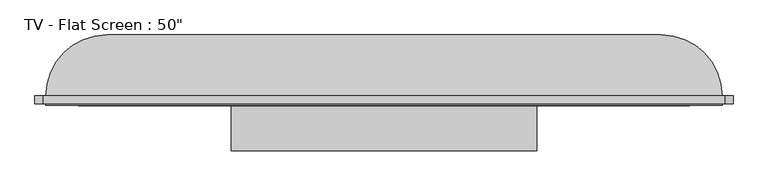
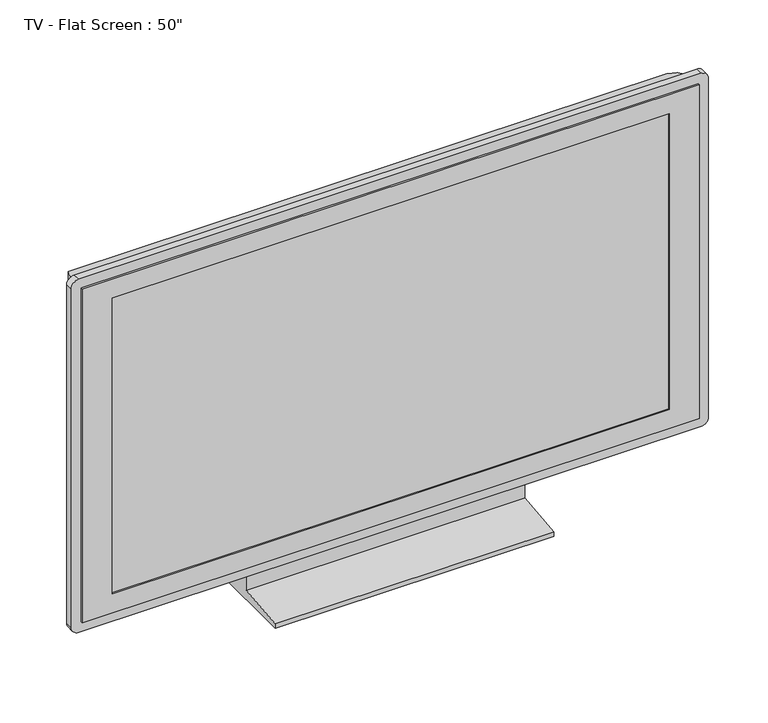
"""IFC4 building model written with IfcOpenShell, lengths in millimetres: furniture geometry."""

from ifc_helpers import new_model, si_unit, point, frame, frame_2d, origin, place, context, project, spatial, polyline, circle_curve, ellipse_curve, trimmed, segment, composite_curve, outline, extrude, faceted_brep, source, transform, mapped, element, save
from ifc_brep_helpers import plane_surface, cylinder_surface, advanced_brep


def furniture_fdf74506(model_context):
    return source(origin(), model_context, "Body", "SolidModel", [
        extrude(outline(polyline([(-51.4613764, 80.0), (-1.4613764, 80.0), (48.5386236, 0.0), (-151.4613764, 0.0), (-151.4613764, 10.0), (-51.4613764, 20.0), (-51.4613764, 80.0)])), frame((-280.6636439, 0.0, 0.0), z_axis=(1.0, 0.0, 0.0), x_axis=(0.0, 1.0, 0.0)), (0.0, 0.0, 1.0), 553.4382596),
        faceted_brep([(609.4937454, -69.4613764, 782.6751733), (-617.3827737, -69.4613764, 782.6751733), (-617.3827737, -69.4613764, 80.0), (609.4937454, -69.4613764, 80.0), (-557.3827737, -69.4613764, 742.6751733), (549.4937454, -69.4613764, 742.6751733), (549.4937454, -69.4613764, 120.0), (-557.3827737, -69.4613764, 120.0), (609.4937454, -51.4613764, 782.6751733), (609.4937454, -51.4613764, 80.0), (-617.3827737, -51.4613764, 80.0), (-617.3827737, -51.4613764, 782.6751733), (-557.3827737, -66.4613764, 742.6751733), (-557.3827737, -66.4613764, 120.0), (549.4937454, -66.4613764, 120.0), (549.4937454, -66.4613764, 742.6751733)], [[[0, 1, 2, 3], [4, 5, 6, 7]], [[8, 9, 10, 11]], [[1, 0, 8, 11]], [[2, 1, 11, 10]], [[3, 2, 10, 9]], [[0, 3, 9, 8]], [[12, 13, 14, 15]], [[12, 15, 5, 4]], [[15, 14, 6, 5]], [[14, 13, 7, 6]], [[13, 12, 4, 7]]]),
        extrude(outline(composite_curve([segment(polyline([(802.6751733, 614.4937454), (802.6751733, -622.3827737)]), True, "CONTINUOUS"), segment(trimmed(circle_curve(frame_2d((787.6751733, -622.3827737)), 15.0), [point((802.6751733, -622.3827737))], [point((787.6751733, -637.3827737))], False, "CARTESIAN"), True, "CONTINUOUS"), segment(polyline([(787.6751733, -637.3827737), (75.0, -637.3827737)]), True, "CONTINUOUS"), segment(trimmed(circle_curve(frame_2d((75.0, -622.3827737)), 15.0), [point((75.0, -637.3827737))], [point((60.0, -622.3827737))], False, "CARTESIAN"), True, "CONTINUOUS"), segment(polyline([(60.0, -622.3827737), (60.0, 614.4937454)]), True, "CONTINUOUS"), segment(trimmed(circle_curve(frame_2d((75.0, 614.4937454)), 15.0), [point((60.0, 614.4937454))], [point((75.0, 629.4937454))], False, "CARTESIAN"), True, "CONTINUOUS"), segment(polyline([(75.0, 629.4937454), (787.6751733, 629.4937454)]), True, "CONTINUOUS"), segment(trimmed(circle_curve(frame_2d((787.6751733, 614.4937454)), 15.0), [point((787.6751733, 629.4937454))], [point((802.6751733, 614.4937454))], False, "CARTESIAN"), True, "CONTINUOUS")], self_intersect=False), holes=[polyline([(782.6751733, 609.4937454), (80.0, 609.4937454), (80.0, -617.3827737), (782.6751733, -617.3827737), (782.6751733, 609.4937454)])]), frame((0.0, -66.4613764, 0.0), z_axis=(0.0, 1.0, 0.0), x_axis=(0.0, 0.0, 1.0)), (0.0, 0.0, 1.0), 15.0),
        advanced_brep(
        [(-617.3827737, -51.4613764, 80.0), (609.4937454, -51.4613764, 80.0), (609.4937454, -51.4613764, 782.6751733), (-617.3827737, -51.4613764, 782.6751733), (499.4937454, 58.5386236, 80.0), (-507.3827737, 58.5386236, 80.0), (-507.3827737, 58.5386236, 672.6751733), (499.4937454, 58.5386236, 672.6751733)],
        [
            (0, 1),
            (1, 2),
            (2, 3),
            (3, 0),
            (4, 5),
            (5, 6),
            (6, 7),
            (7, 4),
            (0, 5, circle_curve(frame((-507.3827737, -51.4613764, 80.0), z_axis=(0.0, 0.0, -1.0), x_axis=(-1.0, 0.0, 0.0)), 110.0)),
            (4, 1, circle_curve(frame((499.4937454, -51.4613764, 80.0), z_axis=(0.0, 0.0, -1.0), x_axis=(1.0, 0.0, 0.0)), 110.0)),
            (7, 2, ellipse_curve(frame((499.4937454, -51.4613764, 672.6751733), z_axis=(0.7071067811865475, 0.0, -0.7071067811865475), x_axis=(0.7071067811865474, 0.0, 0.7071067811865476)), 155.5634919, 110.0)),
            (6, 3, ellipse_curve(frame((-507.3827737, -51.4613764, 672.6751733), z_axis=(0.7071067811865475, 0.0, 0.7071067811865475), x_axis=(-0.7071067811865476, 0.0, 0.7071067811865474)), 155.5634919, 110.0)),
        ],
        [
            plane_surface(frame((-617.3827737, -51.4613764, 782.6751733), z_axis=(0.0, -1.0, 0.0), x_axis=(-1.0, 0.0, 0.0))),
            plane_surface(frame((-617.3827737, 58.5386236, 782.6751733), z_axis=(0.0, 1.0, 0.0), x_axis=(1.0, 0.0, 0.0))),
            plane_surface(frame((-617.3827737, -51.4613764, 80.0), z_axis=(0.0, 0.0, -1.0), x_axis=(0.0, 1.0, 0.0))),
            cylinder_surface(frame((499.4937454, -51.4613764, 80.0), z_axis=(0.0, 0.0, 1.0), x_axis=(1.0, 0.0, 0.0)), 110.0),
            cylinder_surface(frame((609.4937454, -51.4613764, 672.6751733), z_axis=(-1.0, 0.0, 0.0), x_axis=(0.0, 0.0, 1.0)), 110.0),
            cylinder_surface(frame((-507.3827737, -51.4613764, 782.6751733), z_axis=(0.0, 0.0, -1.0), x_axis=(-1.0, 0.0, 0.0)), 110.0),
        ],
        [
            (0, [[1, 2, 3, 4]]),
            (1, [[5, 6, 7, 8]]),
            (2, [[-1, 9, -5, 10]]),
            (3, [[11, -2, -10, -8]]),
            (4, [[-11, -7, 12, -3]]),
            (5, [[-12, -6, -9, -4]]),
        ],
    ),
    ])


if __name__ == "__main__":
    model = new_model("IFC4")
    model_context = context("Model", 3, world=origin())
    ifc_project = project(units=[si_unit("LENGTHUNIT", "METRE", prefix="MILLI")], contexts=[model_context])
    site = spatial("IfcSite", under=ifc_project)
    building = spatial("IfcBuilding", under=site)
    placement = place(None, origin())
    furniture_shape = furniture_fdf74506(model_context)
    element("IfcFurniture", 1, ObjectType="TV - Flat Screen : 50\"", at=placement, inside=building, context=model_context, shape_type="MappedRepresentation", body=[
        mapped(furniture_shape, transform((0.0, 0.0, 0.0), x_axis=(1.0, 0.0, 0.0), y_axis=(0.0, 1.0, 0.0), z_axis=(0.0, 0.0, 1.0))),
    ])
    save(model, "model.ifc")

# Revit data of these elements
# Type "TV - Flat Screen : 50\""
#   SinAng = 0' - 0.0193"
#   L = 3' - 7.57782"
#   H = 2' - 0.51477"
#   Thickness = 0' - 4.33071"
#   Diagonal = 4' - 2"
#   CosAng = 0' - 0.03431"
#   Stand [instance default] = yes
# Element 1 (IfcFurniture, "TV - Flat Screen : 50\"")
#   Materials on its faces: "TV - Black", "TV - Glass", "TV - Screen"
# Materials
#   "TV - Black": class "Miscellaneous", colour RGB 49 49 49, transparency 0
#   "TV - Glass": class "Miscellaneous", colour RGB 157 157 157, transparency 0.9
#   "TV - Screen": class "Miscellaneous", colour RGB 0 0 0, transparency 0
